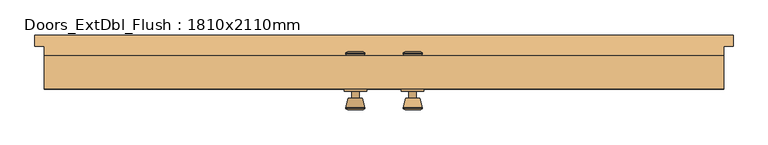
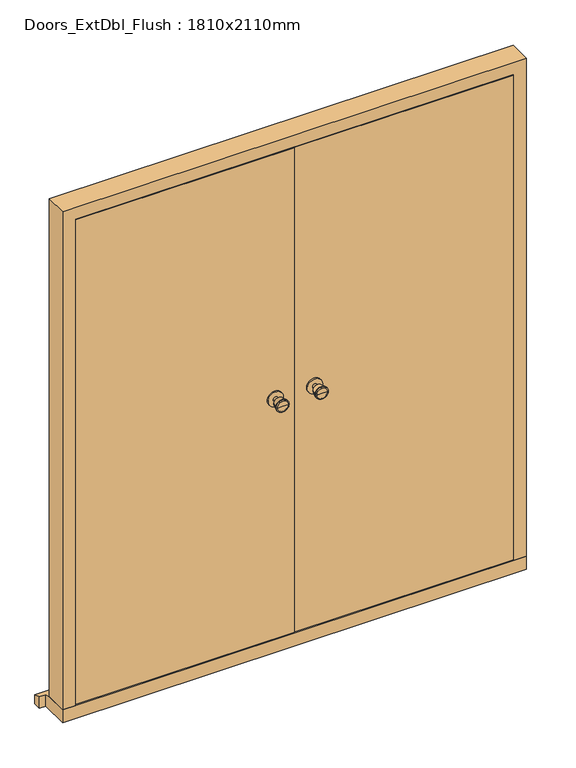
"""IFC4 building model written with IfcOpenShell, lengths in millimetres: door geometry, Doors_ExtDbl_Flush : 1810x2110mm."""

from ifc_helpers import new_model, si_unit, point, frame, frame_2d, origin, place, context, project, spatial, polyline, circle_curve, trimmed, segment, composite_curve, outline, extrude, faceted_brep, source, transform, mapped, element, save
from ifc_brep_helpers import plane_surface, cylinder_surface, revolved_surface, advanced_brep


def doors_extdbl_flush_1810x2110mm_9e9b57c9(model_context):
    return source(origin(), model_context, "Body", "SolidModel", [
        advanced_brep(
        [(-76.5, -5.0, 1050.0), (-66.5, -5.0, 1050.0), (-86.5, -5.0, 1050.0), (-96.9758676, -54.0, 1050.0), (-56.0241324, -54.0, 1050.0), (-76.5, -54.0, 1050.0), (-101.5, -52.1721319, 1050.0), (-51.5, -52.1721319, 1050.0), (-101.5, -48.7084537, 1050.0), (-51.5, -48.7084537, 1050.0), (-95.136236, -24.0, 1050.0), (-57.863764, -24.0, 1050.0), (-86.5, -24.0, 1050.0), (-66.5, -24.0, 1050.0)],
        [
            (0, 1),
            (1, 2, circle_curve(frame((-76.5, -5.0, 1050.0), z_axis=(0.0, 1.0, 0.0), x_axis=(1.0, 0.0, 0.0)), 10.0)),
            (2, 0),
            (2, 1, circle_curve(frame((-76.5, -5.0, 1050.0), z_axis=(0.0, 1.0, 0.0), x_axis=(1.0, 0.0, 0.0)), 10.0)),
            (3, 4, circle_curve(frame((-76.5, -54.0, 1050.0), z_axis=(0.0, -1.0, 0.0), x_axis=(1.0, 0.0, 0.0)), 20.4758676)),
            (4, 5),
            (5, 3),
            (4, 3, circle_curve(frame((-76.5, -54.0, 1050.0), z_axis=(0.0, -1.0, 0.0), x_axis=(1.0, 0.0, 0.0)), 20.4758676)),
            (6, 7, circle_curve(frame((-76.5, -52.1721319, 1050.0), z_axis=(0.0, -1.0, 0.0), x_axis=(1.0, 0.0, 0.0)), 25.0)),
            (7, 4),
            (3, 6),
            (7, 6, circle_curve(frame((-76.5, -52.1721319, 1050.0), z_axis=(0.0, -1.0, 0.0), x_axis=(1.0, 0.0, 0.0)), 25.0)),
            (8, 9, circle_curve(frame((-76.5, -48.7084537, 1050.0), z_axis=(0.0, -1.0, 0.0), x_axis=(1.0, 0.0, 0.0)), 25.0)),
            (9, 7),
            (6, 8),
            (9, 8, circle_curve(frame((-76.5, -48.7084537, 1050.0), z_axis=(0.0, -1.0, 0.0), x_axis=(1.0, 0.0, 0.0)), 25.0)),
            (10, 11, circle_curve(frame((-76.5, -24.0, 1050.0), z_axis=(0.0, -1.0, 0.0), x_axis=(1.0, 0.0, 0.0)), 18.636236)),
            (11, 9),
            (8, 10),
            (11, 10, circle_curve(frame((-76.5, -24.0, 1050.0), z_axis=(0.0, -1.0, 0.0), x_axis=(1.0, 0.0, 0.0)), 18.636236)),
            (12, 13, circle_curve(frame((-76.5, -24.0, 1050.0), z_axis=(0.0, -1.0, 0.0), x_axis=(1.0, 0.0, 0.0)), 10.0)),
            (13, 11),
            (10, 12),
            (13, 12, circle_curve(frame((-76.5, -24.0, 1050.0), z_axis=(0.0, -1.0, 0.0), x_axis=(1.0, 0.0, 0.0)), 10.0)),
            (1, 13),
            (12, 2),
        ],
        [
            plane_surface(frame((-76.5, -5.0, 1050.0), z_axis=(0.0, 1.0, 0.0), x_axis=(1.0, 0.0, 0.0))),
            plane_surface(frame((-76.5, -54.0, 1050.0), z_axis=(0.0, -1.0, 0.0), x_axis=(1.0, 0.0, 0.0))),
            revolved_surface(polyline([(-56.0241324, -54.0, 1050.0), (-51.5, -52.1721319, 1050.0)]), (-76.5, -5.0, 1050.0), (0.0, 1.0, 0.0)),
            cylinder_surface(frame((-76.5, -5.0, 1050.0), z_axis=(0.0, 1.0, 0.0), x_axis=(1.0, 0.0, 0.0)), 25.0),
            revolved_surface(polyline([(-51.5, -48.7084537, 1050.0), (-57.863764, -24.0, 1050.0)]), (-76.5, -5.0, 1050.0), (0.0, 1.0, 0.0)),
            plane_surface(frame((-76.5, -24.0, 1050.0), z_axis=(0.0, 1.0, 0.0), x_axis=(1.0, 0.0, 0.0))),
            cylinder_surface(frame((-76.5, -5.0, 1050.0), z_axis=(0.0, 1.0, 0.0), x_axis=(1.0, 0.0, 0.0)), 10.0),
        ],
        [
            (0, [[1, 2, 3]]),
            (0, [[-3, 4, -1]]),
            (1, [[5, 6, 7]]),
            (1, [[8, -7, -6]]),
            (2, [[9, 10, -5, 11]]),
            (2, [[12, -11, -8, -10]]),
            (3, [[13, 14, -9, 15]]),
            (3, [[16, -15, -12, -14]]),
            (4, [[17, 18, -13, 19]]),
            (4, [[20, -19, -16, -18]]),
            (5, [[21, 22, -17, 23]]),
            (5, [[24, -23, -20, -22]]),
            (6, [[-2, 25, -21, 26]]),
            (6, [[-4, -26, -24, -25]]),
        ],
    ),
        extrude(outline(composite_curve([segment(trimmed(circle_curve(frame_2d((1050.0, -76.5)), 30.0), [point((1050.0, -46.5))], [point((1050.0, -106.5))], False, "CARTESIAN"), True, "CONTINUOUS"), segment(trimmed(circle_curve(frame_2d((1050.0, -76.5)), 30.0), [point((1050.0, -106.5))], [point((1050.0, -46.5))], False, "CARTESIAN"), True, "CONTINUOUS")], self_intersect=False)), frame((0.0, -5.0, 0.0), z_axis=(0.0, 1.0, 0.0), x_axis=(0.0, 0.0, 1.0)), (0.0, 0.0, 1.0), 6.0),
        advanced_brep(
        [(-76.5, 51.0, 1050.0), (-86.5, 51.0, 1050.0), (-66.5, 51.0, 1050.0), (-96.9758676, 100.0, 1050.0), (-76.5, 100.0, 1050.0), (-56.0241324, 100.0, 1050.0), (-101.5, 98.1721319, 1050.0), (-51.5, 98.1721319, 1050.0), (-101.5, 94.7084537, 1050.0), (-51.5, 94.7084537, 1050.0), (-95.136236, 70.0, 1050.0), (-57.863764, 70.0, 1050.0), (-86.5, 70.0, 1050.0), (-66.5, 70.0, 1050.0)],
        [
            (0, 1),
            (1, 2, circle_curve(frame((-76.5, 51.0, 1050.0), z_axis=(0.0, -1.0, 0.0), x_axis=(1.0, 0.0, 0.0)), 10.0)),
            (2, 0),
            (2, 1, circle_curve(frame((-76.5, 51.0, 1050.0), z_axis=(0.0, -1.0, 0.0), x_axis=(1.0, 0.0, 0.0)), 10.0)),
            (3, 4),
            (4, 5),
            (5, 3, circle_curve(frame((-76.5, 100.0, 1050.0), z_axis=(0.0, 1.0, 0.0), x_axis=(1.0, 0.0, 0.0)), 20.4758676)),
            (3, 5, circle_curve(frame((-76.5, 100.0, 1050.0), z_axis=(0.0, 1.0, 0.0), x_axis=(1.0, 0.0, 0.0)), 20.4758676)),
            (6, 3),
            (5, 7),
            (7, 6, circle_curve(frame((-76.5, 98.1721319, 1050.0), z_axis=(0.0, 1.0, 0.0), x_axis=(1.0, 0.0, 0.0)), 25.0)),
            (6, 7, circle_curve(frame((-76.5, 98.1721319, 1050.0), z_axis=(0.0, 1.0, 0.0), x_axis=(1.0, 0.0, 0.0)), 25.0)),
            (8, 6),
            (7, 9),
            (9, 8, circle_curve(frame((-76.5, 94.7084537, 1050.0), z_axis=(0.0, 1.0, 0.0), x_axis=(1.0, 0.0, 0.0)), 25.0)),
            (8, 9, circle_curve(frame((-76.5, 94.7084537, 1050.0), z_axis=(0.0, 1.0, 0.0), x_axis=(1.0, 0.0, 0.0)), 25.0)),
            (10, 8),
            (9, 11),
            (11, 10, circle_curve(frame((-76.5, 70.0, 1050.0), z_axis=(0.0, 1.0, 0.0), x_axis=(1.0, 0.0, 0.0)), 18.636236)),
            (10, 11, circle_curve(frame((-76.5, 70.0, 1050.0), z_axis=(0.0, 1.0, 0.0), x_axis=(1.0, 0.0, 0.0)), 18.636236)),
            (12, 10),
            (11, 13),
            (13, 12, circle_curve(frame((-76.5, 70.0, 1050.0), z_axis=(0.0, 1.0, 0.0), x_axis=(1.0, 0.0, 0.0)), 10.0)),
            (12, 13, circle_curve(frame((-76.5, 70.0, 1050.0), z_axis=(0.0, 1.0, 0.0), x_axis=(1.0, 0.0, 0.0)), 10.0)),
            (1, 12),
            (13, 2),
        ],
        [
            plane_surface(frame((-76.5, 51.0, 1050.0), z_axis=(0.0, -1.0, 0.0), x_axis=(1.0, 0.0, 0.0))),
            plane_surface(frame((-76.5, 100.0, 1050.0), z_axis=(0.0, 1.0, 0.0), x_axis=(1.0, 0.0, 0.0))),
            revolved_surface(polyline([(-56.0241324, 100.0, 1050.0), (-51.5, 98.1721319, 1050.0)]), (-76.5, 51.0, 1050.0), (0.0, -1.0, 0.0)),
            cylinder_surface(frame((-76.5, 51.0, 1050.0), z_axis=(0.0, -1.0, 0.0), x_axis=(1.0, 0.0, 0.0)), 25.0),
            revolved_surface(polyline([(-51.5, 94.7084537, 1050.0), (-57.863764, 70.0, 1050.0)]), (-76.5, 51.0, 1050.0), (0.0, -1.0, 0.0)),
            plane_surface(frame((-76.5, 70.0, 1050.0), z_axis=(0.0, -1.0, 0.0), x_axis=(1.0, 0.0, 0.0))),
            cylinder_surface(frame((-76.5, 51.0, 1050.0), z_axis=(0.0, -1.0, 0.0), x_axis=(1.0, 0.0, 0.0)), 10.0),
        ],
        [
            (0, [[1, 2, 3]]),
            (0, [[-3, 4, -1]]),
            (1, [[5, 6, 7]]),
            (1, [[-6, -5, 8]]),
            (2, [[9, -7, 10, 11]]),
            (2, [[-10, -8, -9, 12]]),
            (3, [[13, -11, 14, 15]]),
            (3, [[-14, -12, -13, 16]]),
            (4, [[17, -15, 18, 19]]),
            (4, [[-18, -16, -17, 20]]),
            (5, [[21, -19, 22, 23]]),
            (5, [[-22, -20, -21, 24]]),
            (6, [[25, -23, 26, -2]]),
            (6, [[-26, -24, -25, -4]]),
        ],
    ),
        extrude(outline(composite_curve([segment(trimmed(circle_curve(frame_2d((1050.0, -76.5)), 30.0), [point((1050.0, -46.5))], [point((1050.0, -106.5))], False, "CARTESIAN"), True, "CONTINUOUS"), segment(trimmed(circle_curve(frame_2d((1050.0, -76.5)), 30.0), [point((1050.0, -106.5))], [point((1050.0, -46.5))], False, "CARTESIAN"), True, "CONTINUOUS")], self_intersect=False)), frame((0.0, 45.0, 0.0), z_axis=(0.0, 1.0, 0.0), x_axis=(0.0, 0.0, 1.0)), (0.0, 0.0, 1.0), 6.0),
        advanced_brep(
        [(76.5, -5.0, 1050.0), (86.5, -5.0, 1050.0), (66.5, -5.0, 1050.0), (96.9758676, -54.0, 1050.0), (76.5, -54.0, 1050.0), (56.0241324, -54.0, 1050.0), (101.5, -52.1721319, 1050.0), (51.5, -52.1721319, 1050.0), (101.5, -48.7084537, 1050.0), (51.5, -48.7084537, 1050.0), (95.136236, -24.0, 1050.0), (57.863764, -24.0, 1050.0), (86.5, -24.0, 1050.0), (66.5, -24.0, 1050.0)],
        [
            (0, 1),
            (1, 2, circle_curve(frame((76.5, -5.0, 1050.0), z_axis=(0.0, 1.0, 0.0), x_axis=(-1.0, 0.0, 0.0)), 10.0)),
            (2, 0),
            (2, 1, circle_curve(frame((76.5, -5.0, 1050.0), z_axis=(0.0, 1.0, 0.0), x_axis=(-1.0, 0.0, 0.0)), 10.0)),
            (3, 4),
            (4, 5),
            (5, 3, circle_curve(frame((76.5, -54.0, 1050.0), z_axis=(0.0, -1.0, 0.0), x_axis=(-1.0, 0.0, 0.0)), 20.4758676)),
            (3, 5, circle_curve(frame((76.5, -54.0, 1050.0), z_axis=(0.0, -1.0, 0.0), x_axis=(-1.0, 0.0, 0.0)), 20.4758676)),
            (6, 3),
            (5, 7),
            (7, 6, circle_curve(frame((76.5, -52.1721319, 1050.0), z_axis=(0.0, -1.0, 0.0), x_axis=(-1.0, 0.0, 0.0)), 25.0)),
            (6, 7, circle_curve(frame((76.5, -52.1721319, 1050.0), z_axis=(0.0, -1.0, 0.0), x_axis=(-1.0, 0.0, 0.0)), 25.0)),
            (8, 6),
            (7, 9),
            (9, 8, circle_curve(frame((76.5, -48.7084537, 1050.0), z_axis=(0.0, -1.0, 0.0), x_axis=(-1.0, 0.0, 0.0)), 25.0)),
            (8, 9, circle_curve(frame((76.5, -48.7084537, 1050.0), z_axis=(0.0, -1.0, 0.0), x_axis=(-1.0, 0.0, 0.0)), 25.0)),
            (10, 8),
            (9, 11),
            (11, 10, circle_curve(frame((76.5, -24.0, 1050.0), z_axis=(0.0, -1.0, 0.0), x_axis=(-1.0, 0.0, 0.0)), 18.636236)),
            (10, 11, circle_curve(frame((76.5, -24.0, 1050.0), z_axis=(0.0, -1.0, 0.0), x_axis=(-1.0, 0.0, 0.0)), 18.636236)),
            (12, 10),
            (11, 13),
            (13, 12, circle_curve(frame((76.5, -24.0, 1050.0), z_axis=(0.0, -1.0, 0.0), x_axis=(-1.0, 0.0, 0.0)), 10.0)),
            (12, 13, circle_curve(frame((76.5, -24.0, 1050.0), z_axis=(0.0, -1.0, 0.0), x_axis=(-1.0, 0.0, 0.0)), 10.0)),
            (1, 12),
            (13, 2),
        ],
        [
            plane_surface(frame((76.5, -5.0, 1050.0), z_axis=(0.0, 1.0, 0.0), x_axis=(-1.0, 0.0, 0.0))),
            plane_surface(frame((76.5, -54.0, 1050.0), z_axis=(0.0, -1.0, 0.0), x_axis=(-1.0, 0.0, 0.0))),
            revolved_surface(polyline([(56.0241324, -54.0, 1050.0), (51.5, -52.1721319, 1050.0)]), (76.5, -5.0, 1050.0), (0.0, 1.0, 0.0)),
            cylinder_surface(frame((76.5, -5.0, 1050.0), z_axis=(0.0, 1.0, 0.0), x_axis=(-1.0, 0.0, 0.0)), 25.0),
            revolved_surface(polyline([(51.5, -48.7084537, 1050.0), (57.863764, -24.0, 1050.0)]), (76.5, -5.0, 1050.0), (0.0, 1.0, 0.0)),
            plane_surface(frame((76.5, -24.0, 1050.0), z_axis=(0.0, 1.0, 0.0), x_axis=(-1.0, 0.0, 0.0))),
            cylinder_surface(frame((76.5, -5.0, 1050.0), z_axis=(0.0, 1.0, 0.0), x_axis=(-1.0, 0.0, 0.0)), 10.0),
        ],
        [
            (0, [[1, 2, 3]]),
            (0, [[-3, 4, -1]]),
            (1, [[5, 6, 7]]),
            (1, [[-6, -5, 8]]),
            (2, [[9, -7, 10, 11]]),
            (2, [[-10, -8, -9, 12]]),
            (3, [[13, -11, 14, 15]]),
            (3, [[-14, -12, -13, 16]]),
            (4, [[17, -15, 18, 19]]),
            (4, [[-18, -16, -17, 20]]),
            (5, [[21, -19, 22, 23]]),
            (5, [[-22, -20, -21, 24]]),
            (6, [[25, -23, 26, -2]]),
            (6, [[-26, -24, -25, -4]]),
        ],
    ),
        extrude(outline(composite_curve([segment(trimmed(circle_curve(frame_2d((1050.0, 76.5)), 30.0), [point((1050.0, 46.5))], [point((1050.0, 106.5))], False, "CARTESIAN"), True, "CONTINUOUS"), segment(trimmed(circle_curve(frame_2d((1050.0, 76.5)), 30.0), [point((1050.0, 106.5))], [point((1050.0, 46.5))], False, "CARTESIAN"), True, "CONTINUOUS")], self_intersect=False)), frame((0.0, -5.0, 0.0), z_axis=(0.0, 1.0, 0.0), x_axis=(0.0, 0.0, 1.0)), (0.0, 0.0, 1.0), 6.0),
        advanced_brep(
        [(76.5, 51.0, 1050.0), (66.5, 51.0, 1050.0), (86.5, 51.0, 1050.0), (96.9758676, 100.0, 1050.0), (56.0241324, 100.0, 1050.0), (76.5, 100.0, 1050.0), (101.5, 98.1721319, 1050.0), (51.5, 98.1721319, 1050.0), (101.5, 94.7084537, 1050.0), (51.5, 94.7084537, 1050.0), (95.136236, 70.0, 1050.0), (57.863764, 70.0, 1050.0), (86.5, 70.0, 1050.0), (66.5, 70.0, 1050.0)],
        [
            (0, 1),
            (1, 2, circle_curve(frame((76.5, 51.0, 1050.0), z_axis=(0.0, -1.0, 0.0), x_axis=(-1.0, 0.0, 0.0)), 10.0)),
            (2, 0),
            (2, 1, circle_curve(frame((76.5, 51.0, 1050.0), z_axis=(0.0, -1.0, 0.0), x_axis=(-1.0, 0.0, 0.0)), 10.0)),
            (3, 4, circle_curve(frame((76.5, 100.0, 1050.0), z_axis=(0.0, 1.0, 0.0), x_axis=(-1.0, 0.0, 0.0)), 20.4758676)),
            (4, 5),
            (5, 3),
            (4, 3, circle_curve(frame((76.5, 100.0, 1050.0), z_axis=(0.0, 1.0, 0.0), x_axis=(-1.0, 0.0, 0.0)), 20.4758676)),
            (6, 7, circle_curve(frame((76.5, 98.1721319, 1050.0), z_axis=(0.0, 1.0, 0.0), x_axis=(-1.0, 0.0, 0.0)), 25.0)),
            (7, 4),
            (3, 6),
            (7, 6, circle_curve(frame((76.5, 98.1721319, 1050.0), z_axis=(0.0, 1.0, 0.0), x_axis=(-1.0, 0.0, 0.0)), 25.0)),
            (8, 9, circle_curve(frame((76.5, 94.7084537, 1050.0), z_axis=(0.0, 1.0, 0.0), x_axis=(-1.0, 0.0, 0.0)), 25.0)),
            (9, 7),
            (6, 8),
            (9, 8, circle_curve(frame((76.5, 94.7084537, 1050.0), z_axis=(0.0, 1.0, 0.0), x_axis=(-1.0, 0.0, 0.0)), 25.0)),
            (10, 11, circle_curve(frame((76.5, 70.0, 1050.0), z_axis=(0.0, 1.0, 0.0), x_axis=(-1.0, 0.0, 0.0)), 18.636236)),
            (11, 9),
            (8, 10),
            (11, 10, circle_curve(frame((76.5, 70.0, 1050.0), z_axis=(0.0, 1.0, 0.0), x_axis=(-1.0, 0.0, 0.0)), 18.636236)),
            (12, 13, circle_curve(frame((76.5, 70.0, 1050.0), z_axis=(0.0, 1.0, 0.0), x_axis=(-1.0, 0.0, 0.0)), 10.0)),
            (13, 11),
            (10, 12),
            (13, 12, circle_curve(frame((76.5, 70.0, 1050.0), z_axis=(0.0, 1.0, 0.0), x_axis=(-1.0, 0.0, 0.0)), 10.0)),
            (1, 13),
            (12, 2),
        ],
        [
            plane_surface(frame((76.5, 51.0, 1050.0), z_axis=(0.0, -1.0, 0.0), x_axis=(-1.0, 0.0, 0.0))),
            plane_surface(frame((76.5, 100.0, 1050.0), z_axis=(0.0, 1.0, 0.0), x_axis=(-1.0, 0.0, 0.0))),
            revolved_surface(polyline([(56.0241324, 100.0, 1050.0), (51.5, 98.1721319, 1050.0)]), (76.5, 51.0, 1050.0), (0.0, -1.0, 0.0)),
            cylinder_surface(frame((76.5, 51.0, 1050.0), z_axis=(0.0, -1.0, 0.0), x_axis=(-1.0, 0.0, 0.0)), 25.0),
            revolved_surface(polyline([(51.5, 94.7084537, 1050.0), (57.863764, 70.0, 1050.0)]), (76.5, 51.0, 1050.0), (0.0, -1.0, 0.0)),
            plane_surface(frame((76.5, 70.0, 1050.0), z_axis=(0.0, -1.0, 0.0), x_axis=(-1.0, 0.0, 0.0))),
            cylinder_surface(frame((76.5, 51.0, 1050.0), z_axis=(0.0, -1.0, 0.0), x_axis=(-1.0, 0.0, 0.0)), 10.0),
        ],
        [
            (0, [[1, 2, 3]]),
            (0, [[-3, 4, -1]]),
            (1, [[5, 6, 7]]),
            (1, [[8, -7, -6]]),
            (2, [[9, 10, -5, 11]]),
            (2, [[12, -11, -8, -10]]),
            (3, [[13, 14, -9, 15]]),
            (3, [[16, -15, -12, -14]]),
            (4, [[17, 18, -13, 19]]),
            (4, [[20, -19, -16, -18]]),
            (5, [[21, 22, -17, 23]]),
            (5, [[24, -23, -20, -22]]),
            (6, [[-2, 25, -21, 26]]),
            (6, [[-4, -26, -24, -25]]),
        ],
    ),
        extrude(outline(composite_curve([segment(trimmed(circle_curve(frame_2d((1050.0, 76.5)), 30.0), [point((1050.0, 46.5))], [point((1050.0, 106.5))], False, "CARTESIAN"), True, "CONTINUOUS"), segment(trimmed(circle_curve(frame_2d((1050.0, 76.5)), 30.0), [point((1050.0, 106.5))], [point((1050.0, 46.5))], False, "CARTESIAN"), True, "CONTINUOUS")], self_intersect=False)), frame((0.0, 45.0, 0.0), z_axis=(0.0, 1.0, 0.0), x_axis=(0.0, 0.0, 1.0)), (0.0, 0.0, 1.0), 6.0),
        faceted_brep([(834.5, 90.0, 54.5), (905.0, 90.0, 54.5), (905.0, 1.0, 54.5), (856.5, 1.0, 54.5), (856.5, 48.0, 54.5), (834.5, 48.0, 54.5), (834.5, 90.0, 2039.5), (-834.5, 90.0, 2039.5), (-834.5, 90.0, 54.5), (-905.0, 90.0, 54.5), (-905.0, 90.0, 2110.0), (905.0, 90.0, 2110.0), (905.0, 1.0, 2110.0), (-905.0, 1.0, 2110.0), (-905.0, 1.0, 54.5), (-856.5, 1.0, 54.5), (-856.5, 1.0, 2061.5), (856.5, 1.0, 2061.5), (856.5, 48.0, 2061.5), (-856.5, 48.0, 2061.5), (-856.5, 48.0, 54.5), (-834.5, 48.0, 54.5), (-834.5, 48.0, 2039.5), (834.5, 48.0, 2039.5)], [[[0, 1, 2, 3, 4, 5]], [[1, 0, 6, 7, 8, 9, 10, 11]], [[2, 1, 11, 12]], [[3, 2, 12, 13, 14, 15, 16, 17]], [[4, 3, 17, 18]], [[5, 4, 18, 19, 20, 21, 22, 23]], [[0, 5, 23, 6]], [[12, 11, 10, 13]], [[18, 17, 16, 19]], [[6, 23, 22, 7]], [[8, 21, 20, 15, 14, 9]], [[13, 10, 9, 14]], [[19, 16, 15, 20]], [[7, 22, 21, 8]]]),
        faceted_brep([(930.0, 145.0, 0.0), (930.0, 145.0, 38.5947221), (930.0, 115.0, 47.2703282), (930.0, 115.0, 0.0), (-930.0, 145.0, 38.5947221), (-930.0, 145.0, 0.0), (-930.0, 115.0, 0.0), (-930.0, 115.0, 47.2703282), (905.0, 115.0, 0.0), (905.0, 1.0, 0.0), (-905.0, 1.0, 0.0), (-905.0, 115.0, 0.0), (-905.0, 115.0, 47.2703282), (-905.0, 90.0, 54.5), (905.0, 90.0, 54.5), (905.0, 115.0, 47.2703282), (-905.0, 1.0, 54.5), (905.0, 1.0, 54.5)], [[[0, 1, 2, 3]], [[4, 5, 6, 7]], [[5, 0, 3, 8, 9, 10, 11, 6]], [[1, 0, 5, 4]], [[1, 4, 7, 12, 13, 14, 15, 2]], [[13, 16, 17, 14]], [[16, 10, 9, 17]], [[12, 11, 10, 16, 13]], [[11, 12, 7, 6]], [[8, 15, 14, 17, 9]], [[15, 8, 3, 2]]]),
        extrude(outline(polyline([(853.5, 1.0), (1.5, 1.0), (1.5, 45.0), (853.5, 45.0), (853.5, 1.0)])), frame((0.0, 0.0, 58.5), z_axis=(0.0, 0.0, 1.0), x_axis=(1.0, 0.0, 0.0)), (0.0, 0.0, 1.0), 2000.0),
        extrude(outline(polyline([(-1.5, 1.0), (-853.5, 1.0), (-853.5, 45.0), (-1.5, 45.0), (-1.5, 1.0)])), frame((0.0, 0.0, 58.5), z_axis=(0.0, 0.0, 1.0), x_axis=(1.0, 0.0, 0.0)), (0.0, 0.0, 1.0), 2000.0),
    ])


if __name__ == "__main__":
    model = new_model("IFC4")
    model_context = context("Model", 3, world=origin())
    ifc_project = project(units=[si_unit("LENGTHUNIT", "METRE", prefix="MILLI")], contexts=[model_context])
    site = spatial("IfcSite", under=ifc_project)
    building = spatial("IfcBuilding", under=site)
    placement = place(None, origin())
    doors_extdbl_flush_1810x2110mm_shape = doors_extdbl_flush_1810x2110mm_9e9b57c9(model_context)
    element("IfcDoor", 1, ObjectType="Doors_ExtDbl_Flush : 1810x2110mm", at=placement, inside=building, context=model_context, shape_type="MappedRepresentation", body=[
        mapped(doors_extdbl_flush_1810x2110mm_shape, transform((0.0, 0.0, 0.0), x_axis=(1.0, 0.0, 0.0), y_axis=(0.0, 1.0, 0.0), z_axis=(0.0, 0.0, 1.0))),
    ])
    save(model, "model.ifc")

# Revit data of these elements
# Type "Doors_ExtDbl_Flush : 1810x2110mm"
#   Type Mark = "44"
#   Type Comments = "External Double"
#   Operation = "DoubleDoorSingleSwing"
#   Keynote = "L20"
#   Analytic Construction = "Metal"
#   Wrap Layers (Ext) from Ext = 102.5 mm
#   Wrap Layers (Int) from Ext = 177.5 mm
#   Thickness = 44 mm
#   Rough Width = 1810 mm
#   Rough Height = 2110 mm
#   O/A Frame Width = 64 mm
#   Heat Transfer Coefficient (U) = 3.7021 W/(m²·K)
#   Handle Z Distance = 1050 mm
#   FrameWidth = 42 mm
#   FrameOffset - External = 25 mm
#   FrameDepth = 89 mm
#   Door Panel Width = 852 mm
#   Door Panel Thickness = 44 mm
#   Door Panel Height = 2000 mm
#   Cill Thickness = 54.5 mm
#   Cill Projection = 30 mm
#   Handle X Distance = 75 mm
#   Height = 2110 mm
#   Structural Tolerance = 6.5 mm
#   Tolerance = 3 mm
#   Undercut = 4 mm
#   Width = 1810 mm
#   Cill Extension = 25 mm
#   Cavity Closer Width = 50 mm
#   Cavity Closer Offset from Ext = 102.5 mm
#   Cavity Closer Depth = 85 mm
#   Define Thermal Properties by = 0
#   Vis - Ironmongery = yes
#   Vis - Cavity Closers = yes
#   Function = 1
#   Material Door = Door - Panel
#   Material Frame = Door - Frame/Mullion
#   Material Ironmongery = Door - Handle
#   Visual Light Transmittance = 0
#   Thermal Resistance (R) = 0
#   Solar Heat Gain Coefficient = 0
#   Wall Closure = (empty or 0)
# Element 1 (IfcDoor, "Doors_ExtDbl_Flush : 1810x2110mm")
#   Materials on its faces: "Door - Handle", "Door - Frame/Mullion", "Door - Panel"
# Materials
#   "Door - Panel": class "Wood", colour RGB 210 159 95, transparency 0, Keynote = "L20", Cost = 0
#   "Door - Frame/Mullion": class "Wood", colour RGB 212 179 113, transparency 0, Keynote = "L20", Cost = 0
#   "Door - Handle": class "Miscellaneous", colour RGB 0 0 0, transparency 0, Keynote = "P21", Cost = 0
